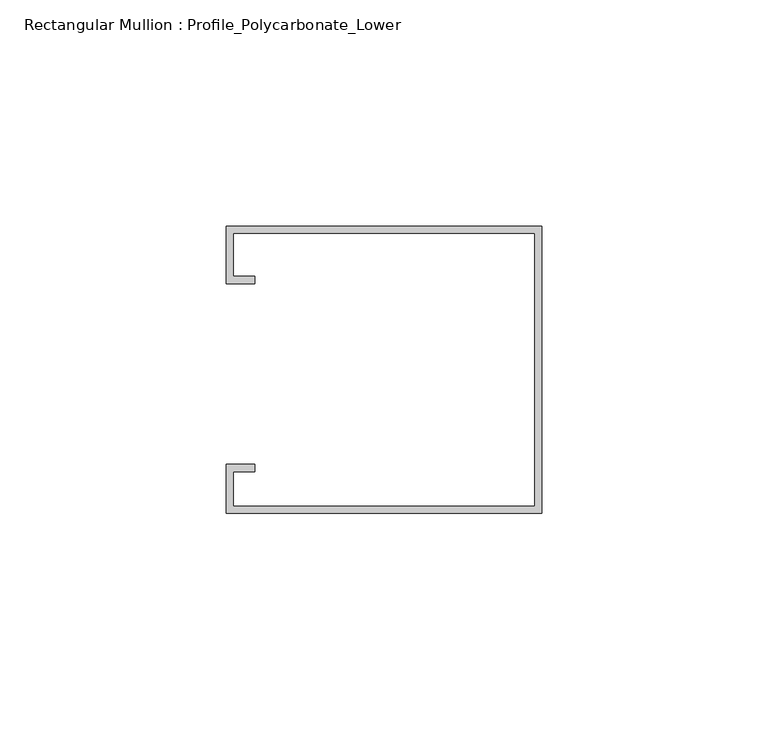
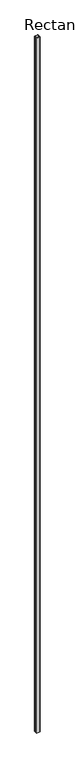
"""IFC4 building model written with IfcOpenShell, lengths in millimetres: member geometry, Rectangular Mullion : Profile_Polycarbonate_Lower."""

from ifc_helpers import new_model, si_unit, frame, origin, place, context, project, spatial, polyline, outline, extrude, source, transform, mapped, element, save


def rectangular_mullion_profile_polycarbonate_lower_7ae10f80(model_context):
    return source(origin(), model_context, "Body", "SweptSolid", [
        extrude(outline(polyline([(0.0, 32.7), (0.0, -30.8), (-69.85, -30.8), (-69.85, -20.0), (-63.5, -20.0), (-63.5, -21.5875), (-68.2625, -21.5875), (-68.2625, -29.2125), (-1.5875, -29.2125), (-1.5875, 31.1125), (-68.2625, 31.1125), (-68.2625, 21.5875), (-63.5, 21.5875), (-63.5, 20.0), (-69.85, 20.0), (-69.85, 32.7), (0.0, 32.7)])), frame((0.0, 0.0, -14490.7), z_axis=(0.0, 0.0, 1.0), x_axis=(1.0, 0.0, 0.0)), (0.0, 0.0, 1.0), 14490.7),
    ])


if __name__ == "__main__":
    model = new_model("IFC4")
    model_context = context("Model", 3, world=origin())
    ifc_project = project(units=[si_unit("LENGTHUNIT", "METRE", prefix="MILLI")], contexts=[model_context])
    site = spatial("IfcSite", under=ifc_project)
    building = spatial("IfcBuilding", under=site)
    placement = place(None, origin())
    rectangular_mullion_profile_polycarbonate_lower_shape = rectangular_mullion_profile_polycarbonate_lower_7ae10f80(model_context)
    element("IfcMember", 1, ObjectType="Rectangular Mullion : Profile_Polycarbonate_Lower", at=placement, inside=building, context=model_context, shape_type="MappedRepresentation", body=[
        mapped(rectangular_mullion_profile_polycarbonate_lower_shape, transform((0.0, 0.0, 0.0), x_axis=(1.0, 0.0, 0.0), y_axis=(0.0, 1.0, 0.0), z_axis=(0.0, 0.0, 1.0))),
    ])
    save(model, "model.ifc")

# Revit data of these elements
# Type "Rectangular Mullion : Profile_Polycarbonate_Lower"
#   built-in parameter 1007322 = 0.208333 (stored number, unit not read)
#   built-in parameter 1007321 = 0 (stored number, unit not read)
#   built-in parameter 1007320 = 0.00520833 (stored number, unit not read)
# Element 1 (IfcMember, "Rectangular Mullion : Profile_Polycarbonate_Lower")
#   Materials on its faces: "ALUMINUM PROFILE AT POLYCARBONATE PANEL"
# Materials
#   "ALUMINUM PROFILE AT POLYCARBONATE PANEL": class "Metal", colour RGB 244 244 244, transparency 0, Description = "Aluminum 6061", Cost = 0
